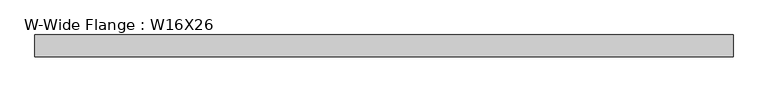
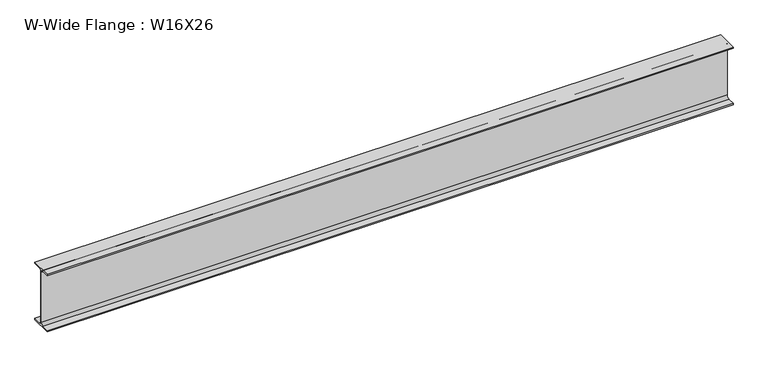
"""IFC4 building model written with IfcOpenShell, lengths in millimetres: beam geometry, W-Wide Flange : W16X26."""

from ifc_helpers import new_model, si_unit, point, frame, frame_2d, origin, place, context, project, spatial, polyline, circle_curve, trimmed, segment, composite_curve, outline, extrude, source, transform, mapped, element, save


def w_wide_flange_w16x26_e29b4586(model_context):
    return source(origin(), model_context, "Body", "SweptSolid", [
        extrude(outline(composite_curve([segment(polyline([(69.85, -190.627), (69.85, -199.39), (-69.85, -199.39), (-69.85, -190.627), (-21.3995, -190.627)]), True, "CONTINUOUS"), segment(trimmed(circle_curve(frame_2d((-21.3995, -172.4025)), 18.2245), [point((-21.3995, -190.627))], [point((-3.175, -172.4025))], True, "CARTESIAN"), True, "CONTINUOUS"), segment(polyline([(-3.175, -172.4025), (-3.175, 172.4025)]), True, "CONTINUOUS"), segment(trimmed(circle_curve(frame_2d((-21.3995, 172.4025)), 18.2245), [point((-3.175, 172.4025))], [point((-21.3995, 190.627))], True, "CARTESIAN"), True, "CONTINUOUS"), segment(polyline([(-21.3995, 190.627), (-69.85, 190.627), (-69.85, 199.39), (69.85, 199.39), (69.85, 190.627), (21.3995, 190.627)]), True, "CONTINUOUS"), segment(trimmed(circle_curve(frame_2d((21.3995, 172.4025)), 18.2245), [point((21.3995, 190.627))], [point((3.175, 172.4025))], True, "CARTESIAN"), True, "CONTINUOUS"), segment(polyline([(3.175, 172.4025), (3.175, -172.4025)]), True, "CONTINUOUS"), segment(trimmed(circle_curve(frame_2d((21.3995, -172.4025)), 18.2245), [point((3.175, -172.4025))], [point((21.3995, -190.627))], True, "CARTESIAN"), True, "CONTINUOUS"), segment(polyline([(21.3995, -190.627), (69.85, -190.627)]), True, "CONTINUOUS")], self_intersect=False)), frame((-2247.9, 0.0, 0.0), z_axis=(1.0, 0.0, 0.0), x_axis=(0.0, 1.0, 0.0)), (0.0, 0.0, 1.0), 4495.8),
    ])


if __name__ == "__main__":
    model = new_model("IFC4")
    model_context = context("Model", 3, world=origin())
    ifc_project = project(units=[si_unit("LENGTHUNIT", "METRE", prefix="MILLI")], contexts=[model_context])
    site = spatial("IfcSite", under=ifc_project)
    building = spatial("IfcBuilding", under=site)
    placement = place(None, origin())
    w_wide_flange_w16x26_shape = w_wide_flange_w16x26_e29b4586(model_context)
    element("IfcBeam", 1, ObjectType="W-Wide Flange : W16X26", at=placement, inside=building, context=model_context, shape_type="MappedRepresentation", body=[
        mapped(w_wide_flange_w16x26_shape, transform((0.0, 0.0, 0.0), x_axis=(1.0, 0.0, 0.0), y_axis=(0.0, 1.0, 0.0), z_axis=(0.0, 0.0, 1.0))),
    ])
    save(model, "model.ifc")

# Revit data of these elements
# Type "W-Wide Flange : W16X26"
#   Assembly Code = "B10"
#   W = 26
#   Length [instance default] = 5' - 0"
#   bf = 0' - 5 1/2"
#   d = 1' - 3.7"
#   k = 0' - 1 1/16"
#   k2 = 0' - 0.7175"
#   tf = 0' - 0.345"
#   tw = 0' - 0 1/4"
#   A = 0.0533333 SF
#   Structural Material [instance default] = Steel ASTM A992
# Element 1 (IfcBeam, "W-Wide Flange : W16X26")
#   Structural Material = Steel ASTM A36
#   Materials on its faces: "Steel ASTM A36"
# Materials
#   "Steel ASTM A992": class "Metal", colour RGB 199 199 199, transparency 0, Description = "Structural steel 50ksi", Cost = 0
#   "Steel ASTM A36": class "Metal", colour RGB 199 199 199, transparency 0, Description = "Structural steel, ASTM A36 Grade B, mill finish", Cost = 0
